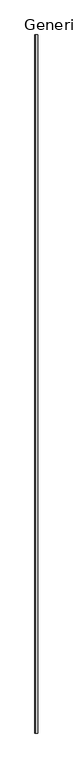
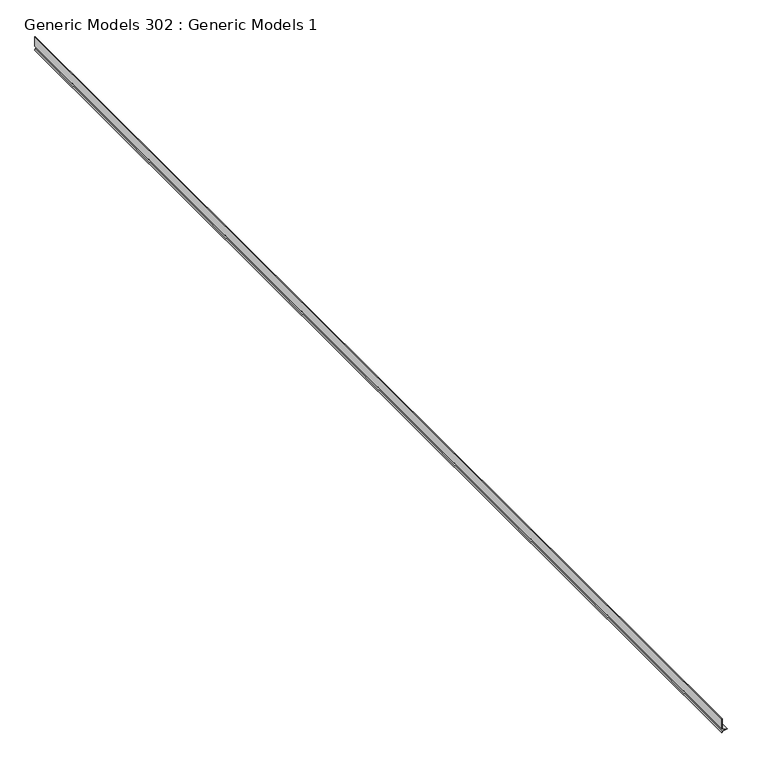
"""IFC4 building model written with IfcOpenShell, lengths in millimetres: proxy geometry, Generic Models 302 : Generic Models 1."""

from ifc_helpers import new_model, si_unit, frame, origin, place, context, project, spatial, polyline, outline, extrude, source, transform, mapped, element, save


def generic_models_302_generic_models_1_98d4aa2f(model_context):
    return source(origin(), model_context, "Body", "SweptSolid", [
        extrude(outline(polyline([(126683.1304643, -9233.0736296), (126689.866, -9254.0286296), (126733.9304643, -9254.0286296), (126733.9304643, -9255.2986296), (126688.9402207, -9255.2986296), (126683.1304643, -9237.2238318), (126677.6303063, -9254.3354345), (126672.5155559, -9255.2986296), (126672.2805244, -9254.050567), (126676.6525161, -9253.2272461), (126683.1304643, -9233.0736296)])), frame((0.0, 6851.0769662, 0.0), z_axis=(0.0, 1.0, 0.0), x_axis=(0.0, 0.0, 1.0)), (0.0, 0.0, 1.0), 5130.8),
    ])


if __name__ == "__main__":
    model = new_model("IFC4")
    model_context = context("Model", 3, world=origin())
    ifc_project = project(units=[si_unit("LENGTHUNIT", "METRE", prefix="MILLI")], contexts=[model_context])
    site = spatial("IfcSite", under=ifc_project)
    building = spatial("IfcBuilding", under=site)
    placement = place(None, origin())
    generic_models_302_generic_models_1_shape = generic_models_302_generic_models_1_98d4aa2f(model_context)
    element("IfcBuildingElementProxy", 1, Name="Generic Models 302 : Generic Models 1", ObjectType="Generic Models 302 : Generic Models 1", at=placement, inside=building, context=model_context, shape_type="MappedRepresentation", body=[
        mapped(generic_models_302_generic_models_1_shape, transform((0.0, 0.0, 0.0), x_axis=(1.0, 0.0, 0.0), y_axis=(0.0, 1.0, 0.0), z_axis=(0.0, 0.0, 1.0))),
    ])
    save(model, "model.ifc")

# Revit data of these elements
# Element 1 (IfcBuildingElementProxy, "Generic Models 302 : Generic Models 1")
#   Materials on its faces: "_16 GA. COPPER WEEP SCREED W/ MIN. 3 1/2\" ATTACHEMENT FLANGE - LAP UNDERLAYMENT OVER WEED SCREED"
# Materials
#   "_16 GA. COPPER WEEP SCREED W/ MIN. 3 1/2\" ATTACHEMENT FLANGE - LAP UNDERLAYMENT OVER WEED SCREED": class "Generic", colour RGB 253 192 103, transparency 0, Cost = 0
